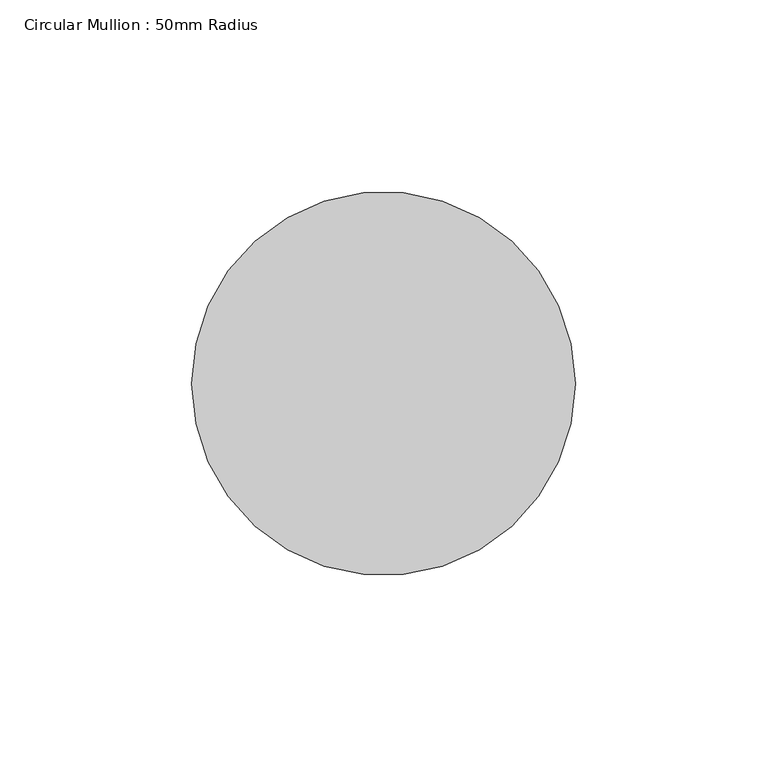
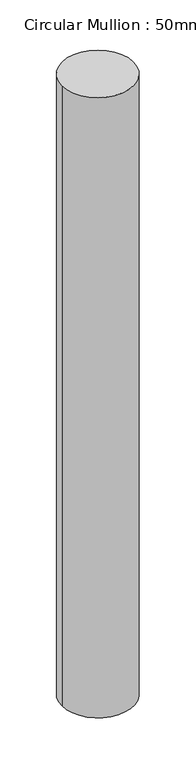
"""IFC4 building model written with IfcOpenShell, lengths in millimetres: member geometry, Circular Mullion : 50mm Radius."""

from ifc_helpers import new_model, si_unit, point, frame, origin, origin_2d, place, context, project, spatial, circle_curve, trimmed, segment, composite_curve, outline, extrude, source, transform, mapped, element, save


def circular_mullion_50mm_radius_a2084d64(model_context):
    return source(origin(), model_context, "Body", "SweptSolid", [
        extrude(outline(composite_curve([segment(trimmed(circle_curve(origin_2d(), 50.0), [point((50.0, 0.0))], [point((-50.0, 0.0))], False, "CARTESIAN"), True, "CONTINUOUS"), segment(trimmed(circle_curve(origin_2d(), 50.0), [point((-50.0, 0.0))], [point((50.0, 0.0))], False, "CARTESIAN"), True, "CONTINUOUS")], self_intersect=False)), frame((0.0, 0.0, -913.5910853), z_axis=(0.0, 0.0, 1.0), x_axis=(1.0, 0.0, 0.0)), (0.0, 0.0, 1.0), 913.5910853),
    ])


if __name__ == "__main__":
    model = new_model("IFC4")
    model_context = context("Model", 3, world=origin())
    ifc_project = project(units=[si_unit("LENGTHUNIT", "METRE", prefix="MILLI")], contexts=[model_context])
    site = spatial("IfcSite", under=ifc_project)
    building = spatial("IfcBuilding", under=site)
    placement = place(None, origin())
    circular_mullion_50mm_radius_shape = circular_mullion_50mm_radius_a2084d64(model_context)
    element("IfcMember", 1, ObjectType="Circular Mullion : 50mm Radius", at=placement, inside=building, context=model_context, shape_type="MappedRepresentation", body=[
        mapped(circular_mullion_50mm_radius_shape, transform((0.0, 0.0, 0.0), x_axis=(1.0, 0.0, 0.0), y_axis=(0.0, 1.0, 0.0), z_axis=(0.0, 0.0, 1.0))),
    ])
    save(model, "model.ifc")

# Revit data of these elements
# Type "Circular Mullion : 50mm Radius"
#   built-in parameter 1007350 = 0.164042 (stored number, unit not read)
# Element 1 (IfcMember, "Circular Mullion : 50mm Radius")
#   Materials on its faces: "Aluminium"
# Materials
#   "Aluminium": class "Metal", colour RGB 247 247 247, transparency 0, Description = "Aluminium 6061", Cost = 0
